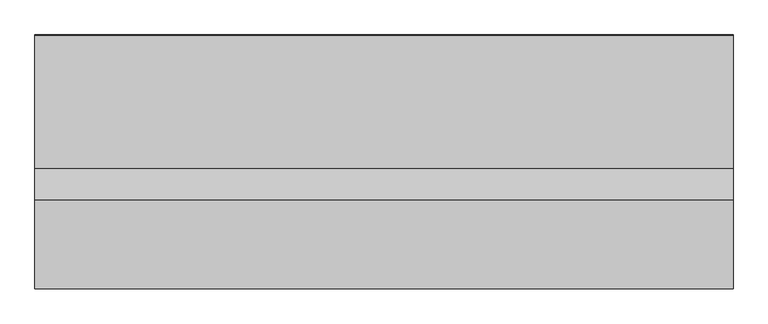
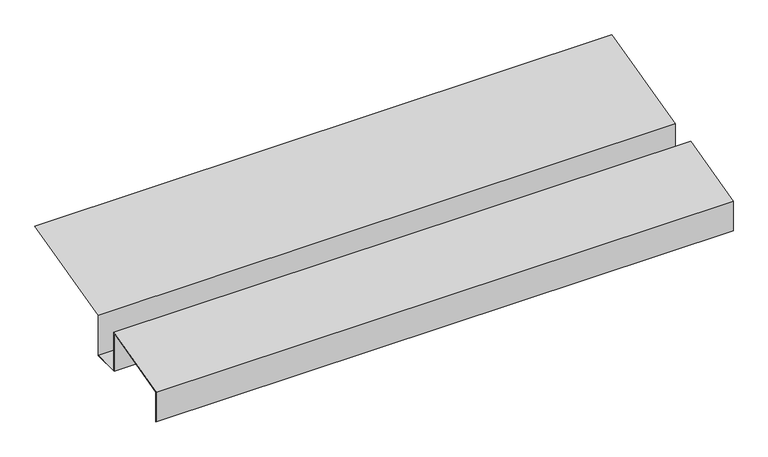
"""IFC4 building model written with IfcOpenShell, lengths in millimetres: proxy geometry, Gutter Adherance Membrane 34392 : Gutter Adherance Membrane 34392."""

import ifcopenshell
import ifcopenshell.guid

model = None  # the IFC model being written
_history = None  # IfcOwnerHistory: only IFC2X3 demands one
_inside = {}  # id of a spatial element -> (the spatial element, [elements in it])
_under = {}  # id of a project, library or spatial element -> (it, [spatial elements below it])
_declared = {}  # id of a project -> (the project, [libraries it declares])
_typed = {}  # id of a type object -> (the type object, [elements of that type])
_made_of = {}  # id of a material, layer set ... -> (it, [elements and type objects made of it])


def new_model(schema):
    """Start an empty IFC model of exactly this schema.

    Asked for "IFC4X3", IfcOpenShell would pick the latest addendum, in which some entities
    have other attributes; the version numbers below select the first issue.
    IFC2X3 requires an IfcOwnerHistory on every rooted entity: one is made here for all.
    """
    global model, _history
    if schema == "IFC4X3":
        model = ifcopenshell.file(schema_version=(4, 3, 0, 0))
    else:
        model = ifcopenshell.file(schema=schema)
    _inside.clear()
    _under.clear()
    _declared.clear()
    _typed.clear()
    _made_of.clear()
    _history = None
    if model.schema == "IFC2X3":
        org = make("IfcOrganization", Name="unknown")
        user = make(
            "IfcPersonAndOrganization",
            ThePerson=make("IfcPerson", FamilyName="unknown"),
            TheOrganization=org,
        )
        app = make(
            "IfcApplication",
            ApplicationDeveloper=org,
            Version="unknown",
            ApplicationFullName="unknown",
            ApplicationIdentifier="unknown",
        )
        _history = make(
            "IfcOwnerHistory",
            OwningUser=user,
            OwningApplication=app,
            ChangeAction="ADDED",
            CreationDate=0,
        )
    return model


def make(cls, **values):
    """One entity of the class cls with the attributes given. An attribute that is None is left unset."""
    return model.create_entity(
        cls, **{name: value for name, value in values.items() if value is not None}
    )


def rooted(cls, **values):
    """An entity with a GlobalId (a new one), such as an element, a storey or a relation."""
    return make(cls, GlobalId=ifcopenshell.guid.new(), OwnerHistory=_history, **values)


def si_unit(unit_type, name, prefix=None):
    """IfcSIUnit, for example si_unit("LENGTHUNIT", "METRE", prefix="MILLI")."""
    return make("IfcSIUnit", UnitType=unit_type, Prefix=prefix, Name=name)


def assignment(units):
    """IfcUnitAssignment: the units of a project."""
    return None if units is None else make("IfcUnitAssignment", Units=units)


def point(xyz):
    """IfcCartesianPoint."""
    return None if xyz is None else make("IfcCartesianPoint", Coordinates=xyz)


def direction(xyz):
    """IfcDirection."""
    return None if xyz is None else make("IfcDirection", DirectionRatios=xyz)


def frame(location, z_axis=None, x_axis=None):
    """IfcAxis2Placement3D, a coordinate frame: its origin and axes. An axis left out is left unset."""
    return make(
        "IfcAxis2Placement3D",
        Location=point(location),
        Axis=direction(z_axis),
        RefDirection=direction(x_axis),
    )


def origin():
    """The frame at (0, 0, 0) with its axes left unset."""
    return frame((0.0, 0.0, 0.0))


def place(relative_to, where):
    """IfcLocalPlacement: puts the frame where relative to a parent placement (None: the world)."""
    return make(
        "IfcLocalPlacement", PlacementRelTo=relative_to, RelativePlacement=where
    )


def context(
    kind, dimensions, precision=None, world=None, true_north=None, identifier=None
):
    """IfcGeometricRepresentationContext, for example the 3D "Model" context."""
    return make(
        "IfcGeometricRepresentationContext",
        ContextIdentifier=identifier,
        ContextType=kind,
        CoordinateSpaceDimension=dimensions,
        Precision=precision,
        WorldCoordinateSystem=world,
        TrueNorth=true_north,
    )


def project(units=None, contexts=None):
    """IfcProject with its units and contexts."""
    return rooted(
        "IfcProject",
        Name="project",
        RepresentationContexts=contexts,
        UnitsInContext=assignment(units),
    )


def spatial(cls, under=None, at=None, **own):
    """A site, building, storey or space (cls), placed at a placement, below another one or the project."""
    s = rooted(cls, ObjectPlacement=at, **own)
    if under is not None:
        _under.setdefault(under.id(), (under, []))[1].append(s)
    return s


def polyline(points):
    """IfcPolyline through the points."""
    return make("IfcPolyline", Points=[point(p) for p in points])


def outline(outer, holes=None, kind="AREA"):
    """IfcArbitraryClosedProfileDef: a profile drawn as a closed curve; with holes, ...WithVoids."""
    if holes is None:
        return make("IfcArbitraryClosedProfileDef", ProfileType=kind, OuterCurve=outer)
    return make(
        "IfcArbitraryProfileDefWithVoids",
        ProfileType=kind,
        OuterCurve=outer,
        InnerCurves=holes,
    )


def extrude(swept, where, along, depth):
    """IfcExtrudedAreaSolid: the profile swept, set in the frame where, extruded along a direction by depth."""
    return make(
        "IfcExtrudedAreaSolid",
        SweptArea=swept,
        Position=where,
        ExtrudedDirection=direction(along),
        Depth=depth,
    )


def shape(context_of_items, identifier, shape_type, items):
    """IfcShapeRepresentation: the items that make up one representation, for example the "Body"."""
    return make(
        "IfcShapeRepresentation",
        ContextOfItems=context_of_items,
        RepresentationIdentifier=identifier,
        RepresentationType=shape_type,
        Items=items,
    )


def source(mapping_origin, context_of_items, identifier, shape_type, items):
    """IfcRepresentationMap: a shape defined once, which mapped items show again and again."""
    return make(
        "IfcRepresentationMap",
        MappingOrigin=mapping_origin,
        MappedRepresentation=shape(context_of_items, identifier, shape_type, items),
    )


def transform(
    local_origin,
    x_axis=None,
    y_axis=None,
    z_axis=None,
    scale=None,
    scale2=None,
    scale3=None,
    uniform=True,
):
    """IfcCartesianTransformationOperator3D, or its non-uniform kind. x_axis, y_axis, z_axis: its Axis1, 2, 3."""
    if uniform:
        return make(
            "IfcCartesianTransformationOperator3D",
            Axis1=direction(x_axis),
            Axis2=direction(y_axis),
            LocalOrigin=point(local_origin),
            Scale=scale,
            Axis3=direction(z_axis),
        )
    return make(
        "IfcCartesianTransformationOperator3DnonUniform",
        Axis1=direction(x_axis),
        Axis2=direction(y_axis),
        LocalOrigin=point(local_origin),
        Scale=scale,
        Axis3=direction(z_axis),
        Scale2=scale2,
        Scale3=scale3,
    )


def mapped(mapping_source, mapping_target):
    """IfcMappedItem: shows the shape of a source again, moved by a transform."""
    return make(
        "IfcMappedItem", MappingSource=mapping_source, MappingTarget=mapping_target
    )


def made_of(thing, what):
    """Note that an element or type object is made of a material, layer set ...; save() writes the relation."""
    if what is not None:
        _made_of.setdefault(what.id(), (what, []))[1].append(thing)
    return thing


def element(
    cls,
    number,
    at=None,
    inside=None,
    cuts=None,
    type_object=None,
    material=None,
    context=None,
    identifier="Body",
    shape_type=None,
    held_by="IfcProductDefinitionShape",
    body=None,
    shapes=None,
    **own,
):
    """One element of the class cls, such as IfcWall. Its Tag is "e" and its number.

    at: its placement. inside: the storey or other place that contains it. cuts: it is an
    opening in that element (IfcRelVoidsElement). A single representation is given by context,
    identifier, shape_type and body (its items); several are given by shapes. held_by: the class
    of the entity that holds the representations. save() writes the other relations.
    """
    e = rooted(cls, Tag="e%d" % number, ObjectPlacement=at, **own)
    if body is not None:
        shapes = [shape(context, identifier, shape_type, body)]
    if shapes is not None:
        e.Representation = make(held_by, Representations=shapes)
    if inside is not None:
        _inside.setdefault(inside.id(), (inside, []))[1].append(e)
    if cuts is not None:
        rooted(
            "IfcRelVoidsElement", RelatingBuildingElement=cuts, RelatedOpeningElement=e
        )
    if type_object is not None:
        _typed.setdefault(type_object.id(), (type_object, []))[1].append(e)
    return made_of(e, material)


def aggregate(whole, parts):
    """IfcRelAggregates: a whole, such as a stair, and the parts it consists of."""
    return rooted("IfcRelAggregates", RelatingObject=whole, RelatedObjects=parts)


def save(model, path):
    """Write the relations noted so far, then the file.

    IfcRelAggregates (storeys below a building ...), IfcRelContainedInSpatialStructure (elements
    in a storey), IfcRelDefinesByType, IfcRelAssociatesMaterial and IfcRelDeclares: one each for
    every whole, place, type object, material and project.
    """
    for whole, parts in _under.values():
        aggregate(whole, parts)
    for where, things in _inside.values():
        rooted(
            "IfcRelContainedInSpatialStructure",
            RelatedElements=things,
            RelatingStructure=where,
        )
    for kind, things in _typed.values():
        rooted("IfcRelDefinesByType", RelatedObjects=things, RelatingType=kind)
    for what, things in _made_of.values():
        rooted("IfcRelAssociatesMaterial", RelatedObjects=things, RelatingMaterial=what)
    for by, libraries in _declared.values():
        rooted("IfcRelDeclares", RelatingContext=by, RelatedDefinitions=libraries)
    model.write(path)


def generic_models_997b00de(model_context):
    return source(origin(), model_context, "Body", "SweptSolid", [
        extrude(outline(polyline([(-5594.6354292, 42634.3617562), (-5594.6354292, 42743.8113639), (-5340.7070312, 42809.4422799), (-5340.7070312, 42668.34375), (-5248.1181651, 42668.34375), (-5248.1181651, 42816.2751118), (-4867.1925603, 42911.3566499), (-4866.8081055, 42909.8164062), (-5246.5306641, 42815.0351562), (-5246.5306641, 42666.75625), (-5342.2945313, 42666.75625), (-5342.2945313, 42807.3923035), (-5593.0479293, 42742.5820053), (-5593.0479293, 42634.3617562), (-5594.6354292, 42634.3617562)])), frame((12382.7678845, 0.0, 0.0), z_axis=(1.0, 0.0, 0.0), x_axis=(0.0, 1.0, 0.0)), (0.0, 0.0, 1.0), 2000.25),
    ])


if __name__ == "__main__":
    model = new_model("IFC4")
    model_context = context("Model", 3, world=origin())
    ifc_project = project(units=[si_unit("LENGTHUNIT", "METRE", prefix="MILLI")], contexts=[model_context])
    site = spatial("IfcSite", under=ifc_project)
    building = spatial("IfcBuilding", under=site)
    placement = place(None, origin())
    generic_models_shape = generic_models_997b00de(model_context)
    element("IfcBuildingElementProxy", 1, Name="Gutter Adherance Membrane 34392 : Gutter Adherance Membrane 34392", ObjectType="Gutter Adherance Membrane 34392 : Gutter Adherance Membrane 34392", at=placement, inside=building, context=model_context, shape_type="MappedRepresentation", body=[
        mapped(generic_models_shape, transform((0.0, 0.0, 0.0), x_axis=(1.0, 0.0, 0.0), y_axis=(0.0, 1.0, 0.0), z_axis=(0.0, 0.0, 1.0))),
    ])
    save(model, "model.ifc")

# Revit data of these elements
# Type "Gutter Adherance Membrane 34392 : Gutter Adherance Membrane 34392"
#   NameOverride = "Gutter Adherance Membrane"
# Element 1 (IfcBuildingElementProxy, "Gutter Adherance Membrane 34392 : Gutter Adherance Membrane 34392")
#   Materials on its faces: "SELF ADHERED MEMBRANE W/ END DAMS WHERE POSSIBLE"
# Materials
#   "SELF ADHERED MEMBRANE W/ END DAMS WHERE POSSIBLE": class "Unassigned", colour RGB 255 255 127, transparency 0
